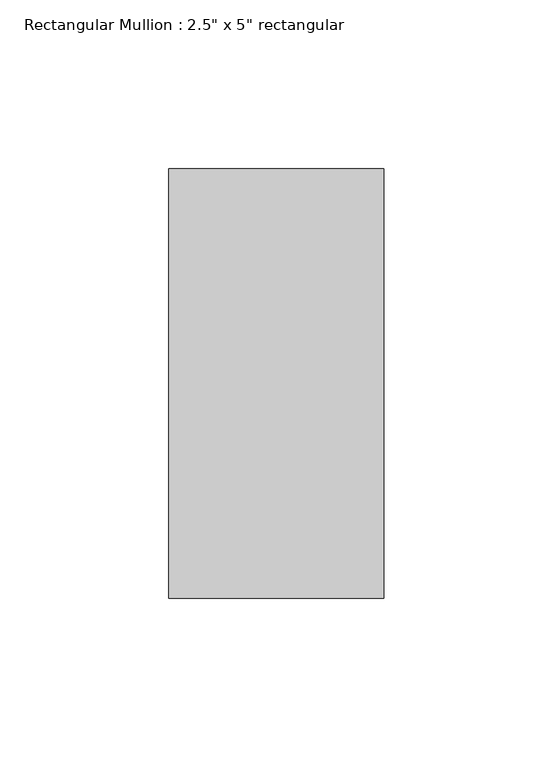
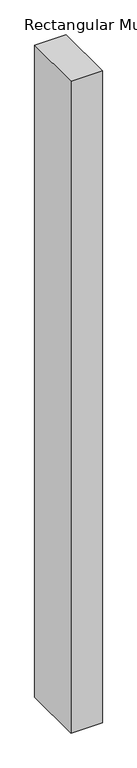
"""IFC4 building model written with IfcOpenShell, lengths in millimetres: member geometry."""

import ifcopenshell
import ifcopenshell.guid

model = None  # the IFC model being written
_history = None  # IfcOwnerHistory: only IFC2X3 demands one
_inside = {}  # id of a spatial element -> (the spatial element, [elements in it])
_under = {}  # id of a project, library or spatial element -> (it, [spatial elements below it])
_declared = {}  # id of a project -> (the project, [libraries it declares])
_typed = {}  # id of a type object -> (the type object, [elements of that type])
_made_of = {}  # id of a material, layer set ... -> (it, [elements and type objects made of it])


def new_model(schema):
    """Start an empty IFC model of exactly this schema.

    Asked for "IFC4X3", IfcOpenShell would pick the latest addendum, in which some entities
    have other attributes; the version numbers below select the first issue.
    IFC2X3 requires an IfcOwnerHistory on every rooted entity: one is made here for all.
    """
    global model, _history
    if schema == "IFC4X3":
        model = ifcopenshell.file(schema_version=(4, 3, 0, 0))
    else:
        model = ifcopenshell.file(schema=schema)
    _inside.clear()
    _under.clear()
    _declared.clear()
    _typed.clear()
    _made_of.clear()
    _history = None
    if model.schema == "IFC2X3":
        org = make("IfcOrganization", Name="unknown")
        user = make(
            "IfcPersonAndOrganization",
            ThePerson=make("IfcPerson", FamilyName="unknown"),
            TheOrganization=org,
        )
        app = make(
            "IfcApplication",
            ApplicationDeveloper=org,
            Version="unknown",
            ApplicationFullName="unknown",
            ApplicationIdentifier="unknown",
        )
        _history = make(
            "IfcOwnerHistory",
            OwningUser=user,
            OwningApplication=app,
            ChangeAction="ADDED",
            CreationDate=0,
        )
    return model


def make(cls, **values):
    """One entity of the class cls with the attributes given. An attribute that is None is left unset."""
    return model.create_entity(
        cls, **{name: value for name, value in values.items() if value is not None}
    )


def rooted(cls, **values):
    """An entity with a GlobalId (a new one), such as an element, a storey or a relation."""
    return make(cls, GlobalId=ifcopenshell.guid.new(), OwnerHistory=_history, **values)


def si_unit(unit_type, name, prefix=None):
    """IfcSIUnit, for example si_unit("LENGTHUNIT", "METRE", prefix="MILLI")."""
    return make("IfcSIUnit", UnitType=unit_type, Prefix=prefix, Name=name)


def assignment(units):
    """IfcUnitAssignment: the units of a project."""
    return None if units is None else make("IfcUnitAssignment", Units=units)


def point(xyz):
    """IfcCartesianPoint."""
    return None if xyz is None else make("IfcCartesianPoint", Coordinates=xyz)


def direction(xyz):
    """IfcDirection."""
    return None if xyz is None else make("IfcDirection", DirectionRatios=xyz)


def frame(location, z_axis=None, x_axis=None):
    """IfcAxis2Placement3D, a coordinate frame: its origin and axes. An axis left out is left unset."""
    return make(
        "IfcAxis2Placement3D",
        Location=point(location),
        Axis=direction(z_axis),
        RefDirection=direction(x_axis),
    )


def origin():
    """The frame at (0, 0, 0) with its axes left unset."""
    return frame((0.0, 0.0, 0.0))


def place(relative_to, where):
    """IfcLocalPlacement: puts the frame where relative to a parent placement (None: the world)."""
    return make(
        "IfcLocalPlacement", PlacementRelTo=relative_to, RelativePlacement=where
    )


def context(
    kind, dimensions, precision=None, world=None, true_north=None, identifier=None
):
    """IfcGeometricRepresentationContext, for example the 3D "Model" context."""
    return make(
        "IfcGeometricRepresentationContext",
        ContextIdentifier=identifier,
        ContextType=kind,
        CoordinateSpaceDimension=dimensions,
        Precision=precision,
        WorldCoordinateSystem=world,
        TrueNorth=true_north,
    )


def project(units=None, contexts=None):
    """IfcProject with its units and contexts."""
    return rooted(
        "IfcProject",
        Name="project",
        RepresentationContexts=contexts,
        UnitsInContext=assignment(units),
    )


def spatial(cls, under=None, at=None, **own):
    """A site, building, storey or space (cls), placed at a placement, below another one or the project."""
    s = rooted(cls, ObjectPlacement=at, **own)
    if under is not None:
        _under.setdefault(under.id(), (under, []))[1].append(s)
    return s


def polyline(points):
    """IfcPolyline through the points."""
    return make("IfcPolyline", Points=[point(p) for p in points])


def outline(outer, holes=None, kind="AREA"):
    """IfcArbitraryClosedProfileDef: a profile drawn as a closed curve; with holes, ...WithVoids."""
    if holes is None:
        return make("IfcArbitraryClosedProfileDef", ProfileType=kind, OuterCurve=outer)
    return make(
        "IfcArbitraryProfileDefWithVoids",
        ProfileType=kind,
        OuterCurve=outer,
        InnerCurves=holes,
    )


def extrude(swept, where, along, depth):
    """IfcExtrudedAreaSolid: the profile swept, set in the frame where, extruded along a direction by depth."""
    return make(
        "IfcExtrudedAreaSolid",
        SweptArea=swept,
        Position=where,
        ExtrudedDirection=direction(along),
        Depth=depth,
    )


def shape(context_of_items, identifier, shape_type, items):
    """IfcShapeRepresentation: the items that make up one representation, for example the "Body"."""
    return make(
        "IfcShapeRepresentation",
        ContextOfItems=context_of_items,
        RepresentationIdentifier=identifier,
        RepresentationType=shape_type,
        Items=items,
    )


def source(mapping_origin, context_of_items, identifier, shape_type, items):
    """IfcRepresentationMap: a shape defined once, which mapped items show again and again."""
    return make(
        "IfcRepresentationMap",
        MappingOrigin=mapping_origin,
        MappedRepresentation=shape(context_of_items, identifier, shape_type, items),
    )


def transform(
    local_origin,
    x_axis=None,
    y_axis=None,
    z_axis=None,
    scale=None,
    scale2=None,
    scale3=None,
    uniform=True,
):
    """IfcCartesianTransformationOperator3D, or its non-uniform kind. x_axis, y_axis, z_axis: its Axis1, 2, 3."""
    if uniform:
        return make(
            "IfcCartesianTransformationOperator3D",
            Axis1=direction(x_axis),
            Axis2=direction(y_axis),
            LocalOrigin=point(local_origin),
            Scale=scale,
            Axis3=direction(z_axis),
        )
    return make(
        "IfcCartesianTransformationOperator3DnonUniform",
        Axis1=direction(x_axis),
        Axis2=direction(y_axis),
        LocalOrigin=point(local_origin),
        Scale=scale,
        Axis3=direction(z_axis),
        Scale2=scale2,
        Scale3=scale3,
    )


def mapped(mapping_source, mapping_target):
    """IfcMappedItem: shows the shape of a source again, moved by a transform."""
    return make(
        "IfcMappedItem", MappingSource=mapping_source, MappingTarget=mapping_target
    )


def made_of(thing, what):
    """Note that an element or type object is made of a material, layer set ...; save() writes the relation."""
    if what is not None:
        _made_of.setdefault(what.id(), (what, []))[1].append(thing)
    return thing


def element(
    cls,
    number,
    at=None,
    inside=None,
    cuts=None,
    type_object=None,
    material=None,
    context=None,
    identifier="Body",
    shape_type=None,
    held_by="IfcProductDefinitionShape",
    body=None,
    shapes=None,
    **own,
):
    """One element of the class cls, such as IfcWall. Its Tag is "e" and its number.

    at: its placement. inside: the storey or other place that contains it. cuts: it is an
    opening in that element (IfcRelVoidsElement). A single representation is given by context,
    identifier, shape_type and body (its items); several are given by shapes. held_by: the class
    of the entity that holds the representations. save() writes the other relations.
    """
    e = rooted(cls, Tag="e%d" % number, ObjectPlacement=at, **own)
    if body is not None:
        shapes = [shape(context, identifier, shape_type, body)]
    if shapes is not None:
        e.Representation = make(held_by, Representations=shapes)
    if inside is not None:
        _inside.setdefault(inside.id(), (inside, []))[1].append(e)
    if cuts is not None:
        rooted(
            "IfcRelVoidsElement", RelatingBuildingElement=cuts, RelatedOpeningElement=e
        )
    if type_object is not None:
        _typed.setdefault(type_object.id(), (type_object, []))[1].append(e)
    return made_of(e, material)


def aggregate(whole, parts):
    """IfcRelAggregates: a whole, such as a stair, and the parts it consists of."""
    return rooted("IfcRelAggregates", RelatingObject=whole, RelatedObjects=parts)


def save(model, path):
    """Write the relations noted so far, then the file.

    IfcRelAggregates (storeys below a building ...), IfcRelContainedInSpatialStructure (elements
    in a storey), IfcRelDefinesByType, IfcRelAssociatesMaterial and IfcRelDeclares: one each for
    every whole, place, type object, material and project.
    """
    for whole, parts in _under.values():
        aggregate(whole, parts)
    for where, things in _inside.values():
        rooted(
            "IfcRelContainedInSpatialStructure",
            RelatedElements=things,
            RelatingStructure=where,
        )
    for kind, things in _typed.values():
        rooted("IfcRelDefinesByType", RelatedObjects=things, RelatingType=kind)
    for what, things in _made_of.values():
        rooted("IfcRelAssociatesMaterial", RelatedObjects=things, RelatingMaterial=what)
    for by, libraries in _declared.values():
        rooted("IfcRelDeclares", RelatingContext=by, RelatedDefinitions=libraries)
    model.write(path)


def member_0e9192ed(model_context):
    return source(origin(), model_context, "Body", "SweptSolid", [
        extrude(outline(polyline([(31.75, 63.5), (31.75, -63.5), (-31.75, -63.5), (-31.75, 63.5), (31.75, 63.5)])), frame((0.0, 0.0, -1394.8833336), z_axis=(0.0, 0.0, 1.0), x_axis=(1.0, 0.0, 0.0)), (0.0, 0.0, 1.0), 1394.8833336),
    ])


if __name__ == "__main__":
    model = new_model("IFC4")
    model_context = context("Model", 3, world=origin())
    ifc_project = project(units=[si_unit("LENGTHUNIT", "METRE", prefix="MILLI")], contexts=[model_context])
    site = spatial("IfcSite", under=ifc_project)
    building = spatial("IfcBuilding", under=site)
    placement = place(None, origin())
    member_shape = member_0e9192ed(model_context)
    element("IfcMember", 1, ObjectType="Rectangular Mullion : 2.5\" x 5\" rectangular", at=placement, inside=building, context=model_context, shape_type="MappedRepresentation", body=[
        mapped(member_shape, transform((0.0, 0.0, 0.0), x_axis=(1.0, 0.0, 0.0), y_axis=(0.0, 1.0, 0.0), z_axis=(0.0, 0.0, 1.0))),
    ])
    save(model, "model.ifc")

# Revit data of these elements
# Project information
#   Organization Name = "G3B Press"
#   Organization Description = "Paul F. Aubin Cosulting Services, Inc."
#   Building Name = "Revit Essentials for Architecture"
#   Author = "Paul F. Aubin"
#   Author Website = "https://www.paulaubin.com"
#   Copyright = "Copyright © 2020 Paul F Aubin, all rights reserved"
#   Design Option = "Main Model"
#   Project Issue Date = "8/1/2020"
#   Project Status = "Design Development"
#   Client Name = "Printing and Output"
#   Project Address = "123 State ST\nSuite 301\nChicago, IL 60606"
#   Project Name = "15 Commercial"
#   Project Number = "2020.04A"
# Type "Rectangular Mullion : 2.5\" x 5\" rectangular"
#   built-in parameter 1007304 = 0.416667 (stored number, unit not read)
#   built-in parameter 1007301 = 0.104167 (stored number, unit not read)
#   built-in parameter 1007300 = 0.104167 (stored number, unit not read)
# Element 1 (IfcMember, "Rectangular Mullion : 2.5\" x 5\" rectangular")
#   Materials on its faces: "Aluminum"
# Materials
#   "Aluminum": class "Metal", colour RGB 247 247 247, transparency 0, Description = "Aluminum 6061", Cost = 0
